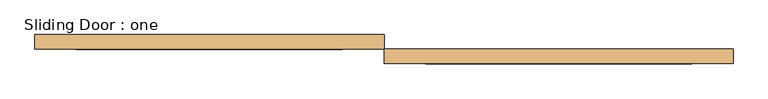
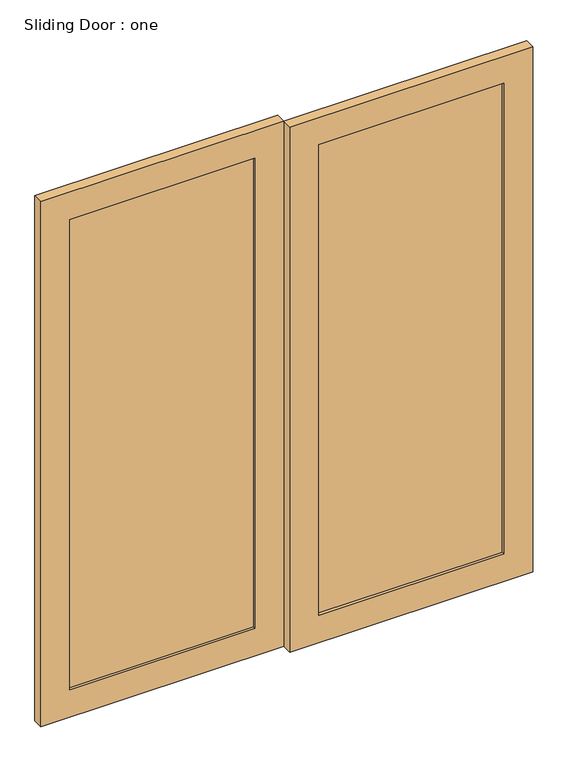
"""IFC4 building model written with IfcOpenShell, lengths in millimetres: door geometry, Sliding Door : one."""

from ifc_helpers import new_model, si_unit, frame, origin, place, context, project, spatial, polyline, outline, extrude, source, transform, mapped, element, save


def sliding_door_one_d40f44c8(model_context):
    return source(origin(), model_context, "Body", "SweptSolid", [
        extrude(outline(polyline([(-127.0, 50.8), (-127.0, 31.75), (-939.8, 31.75), (-939.8, 50.8), (-127.0, 50.8)])), frame((0.0, 0.0, 127.0), z_axis=(0.0, 0.0, 1.0), x_axis=(1.0, 0.0, 0.0)), (0.0, 0.0, 1.0), 2184.4),
        extrude(outline(polyline([(939.8, 6.35), (939.8, -12.7), (127.0, -12.7), (127.0, 6.35), (939.8, 6.35)])), frame((0.0, 0.0, 127.0), z_axis=(0.0, 0.0, 1.0), x_axis=(1.0, 0.0, 0.0)), (0.0, 0.0, 1.0), 2184.4),
        extrude(outline(polyline([(2438.4, -1066.8), (0.0, -1066.8), (0.0, 0.0), (2438.4, 0.0), (2438.4, -1066.8)]), holes=[polyline([(127.0, -127.0), (127.0, -939.8), (2311.4, -939.8), (2311.4, -127.0), (127.0, -127.0)])]), frame((0.0, 19.05, 0.0), z_axis=(0.0, 1.0, 0.0), x_axis=(0.0, 0.0, 1.0)), (0.0, 0.0, 1.0), 44.45),
        extrude(outline(polyline([(2438.4, 0.0), (0.0, 0.0), (0.0, 1066.8), (2438.4, 1066.8), (2438.4, 0.0)]), holes=[polyline([(127.0, 939.8), (127.0, 127.0), (2311.4, 127.0), (2311.4, 939.8), (127.0, 939.8)])]), frame((0.0, -25.4, 0.0), z_axis=(0.0, 1.0, 0.0), x_axis=(0.0, 0.0, 1.0)), (0.0, 0.0, 1.0), 44.45),
    ])


if __name__ == "__main__":
    model = new_model("IFC4")
    model_context = context("Model", 3, world=origin())
    ifc_project = project(units=[si_unit("LENGTHUNIT", "METRE", prefix="MILLI")], contexts=[model_context])
    site = spatial("IfcSite", under=ifc_project)
    building = spatial("IfcBuilding", under=site)
    placement = place(None, origin())
    sliding_door_one_shape = sliding_door_one_d40f44c8(model_context)
    element("IfcDoor", 1, ObjectType="Sliding Door : one", at=placement, inside=building, context=model_context, shape_type="MappedRepresentation", body=[
        mapped(sliding_door_one_shape, transform((0.0, 0.0, 0.0), x_axis=(1.0, 0.0, 0.0), y_axis=(0.0, 1.0, 0.0), z_axis=(0.0, 0.0, 1.0))),
    ])
    save(model, "model.ifc")

# Revit data of these elements
# Type "Sliding Door : one"
#   Type Mark = "42"
#   Analytic Construction = "<None>"
#   Stile_Width = 0' - 5"
#   Door_Thickness = 0' - 1 3/4"
#   Door_Offset = 0' - 1"
#   Glass_Material = SAFETY GLAZING
#   Frame_Material = INTERIOR GRADE ALUMINUM STOREFRONT W/ SAFETY GLAZING
#   Function = (empty or 0)
# Element 1 (IfcDoor, "Sliding Door : one")
#   Materials on its faces: "INTERIOR GRADE ALUMINUM STOREFRONT W/ SAFETY GLAZING", "SAFETY GLAZING"
# Materials
#   "SAFETY GLAZING": class "Glass", colour RGB 142 168 196, transparency 0.75, Description = "Soda Lime Glass", Cost = 0
#   "INTERIOR GRADE ALUMINUM STOREFRONT W/ SAFETY GLAZING": class "Metal", colour RGB 226 226 226, transparency 0, Description = "Aluminum 6061", Cost = 0
